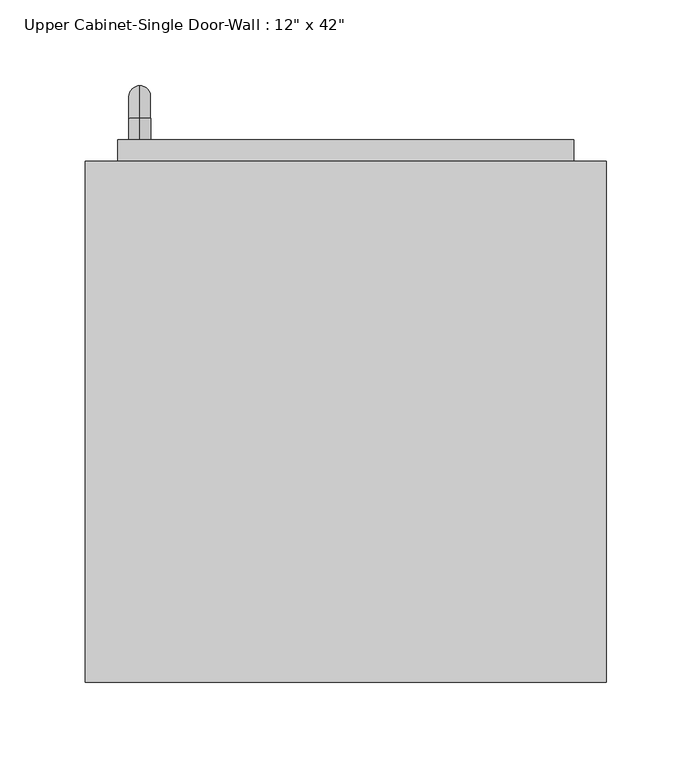
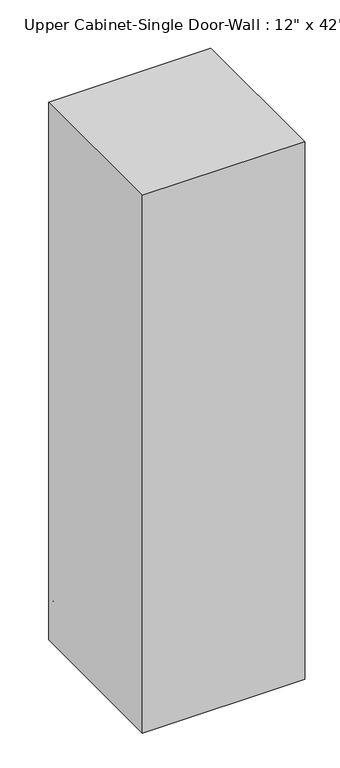
"""IFC4 building model written with IfcOpenShell, lengths in millimetres: furniture geometry."""

from ifc_helpers import new_model, si_unit, point, frame, origin, place, context, project, spatial, polyline, circle_curve, ellipse_curve, trimmed, outline, extrude, faceted_brep, source, transform, mapped, element, save
from ifc_brep_helpers import plane_surface, cylinder_surface, revolved_surface, advanced_brep


def furniture_aa269a34(model_context):
    return source(origin(), model_context, "Body", "SolidModel", [
        faceted_brep([(-122.6288372, 80.9625, 2438.4), (-122.6288372, 80.9625, 1371.6), (182.1711628, 80.9625, 1371.6), (182.1711628, 80.9625, 2438.4), (-122.6288372, 385.7625, 2438.4), (182.1711628, 385.7625, 2438.4), (182.1711628, 385.7625, 1371.6), (-122.6288372, 385.7625, 1371.6), (-103.5788372, 385.7625, 2419.35), (-103.5788372, 385.7625, 1390.65), (163.1211628, 385.7625, 1390.65), (163.1211628, 385.7625, 2419.35), (163.1211628, 100.0125, 2419.35), (-103.5788372, 100.0125, 2419.35), (163.1211628, 100.0125, 1390.65), (-103.5788372, 100.0125, 1390.65)], [[[0, 1, 2, 3]], [[4, 5, 6, 7], [8, 9, 10, 11]], [[1, 0, 4, 7]], [[2, 1, 7, 6]], [[3, 2, 6, 5]], [[0, 3, 5, 4]], [[8, 11, 12, 13]], [[11, 10, 14, 12]], [[10, 9, 15, 14]], [[9, 8, 13, 15]], [[13, 12, 14, 15]]]),
        advanced_brep(
        [(-90.8788372, 398.4625, 1517.65), (-90.8788372, 398.4625, 1530.35), (-90.8788372, 411.1625, 1517.65), (-90.8788372, 411.1625, 1530.35), (-90.8788372, 430.2125, 1511.3), (-90.8788372, 417.5125, 1511.3), (-90.8788372, 417.5125, 1435.1), (-90.8788372, 430.2125, 1435.1), (-90.8788372, 411.1625, 1416.05), (-90.8788372, 411.1625, 1428.75), (-90.8788372, 398.4625, 1428.75), (-90.8788372, 398.4625, 1416.05)],
        [
            (0, 1, circle_curve(frame((-90.8788372, 398.4625, 1524.0), z_axis=(0.0, -1.0, 0.0), x_axis=(0.0, 0.0, 1.0)), 6.35)),
            (1, 0, circle_curve(frame((-90.8788372, 398.4625, 1524.0), z_axis=(0.0, -1.0, 0.0), x_axis=(0.0, 0.0, 1.0)), 6.35)),
            (0, 2),
            (2, 3, circle_curve(frame((-90.8788372, 411.1625, 1524.0), z_axis=(0.0, -1.0, 0.0), x_axis=(0.0, 0.0, 1.0)), 6.35)),
            (3, 1),
            (3, 2, circle_curve(frame((-90.8788372, 411.1625, 1524.0), z_axis=(0.0, -1.0, 0.0), x_axis=(0.0, 0.0, 1.0)), 6.35)),
            (4, 3, circle_curve(frame((-90.8788372, 411.1625, 1511.3), z_axis=(1.0, 0.0, 0.0), x_axis=(0.0, 0.0, 1.0)), 19.05)),
            (2, 5, circle_curve(frame((-90.8788372, 411.1625, 1511.3), z_axis=(-1.0, 0.0, 0.0), x_axis=(0.0, 0.0, 1.0)), 6.35)),
            (5, 4, circle_curve(frame((-90.8788372, 423.8625, 1511.3), z_axis=(0.0, 0.0, 1.0), x_axis=(0.0, 1.0, 0.0)), 6.35)),
            (4, 5, circle_curve(frame((-90.8788372, 423.8625, 1511.3), z_axis=(0.0, 0.0, 1.0), x_axis=(0.0, 1.0, 0.0)), 6.35)),
            (5, 6),
            (6, 7, circle_curve(frame((-90.8788372, 423.8625, 1435.1), z_axis=(0.0, 0.0, 1.0), x_axis=(0.0, 1.0, 0.0)), 6.35)),
            (7, 4),
            (7, 6, circle_curve(frame((-90.8788372, 423.8625, 1435.1), z_axis=(0.0, 0.0, 1.0), x_axis=(0.0, 1.0, 0.0)), 6.35)),
            (8, 7, circle_curve(frame((-90.8788372, 411.1625, 1435.1), z_axis=(1.0, 0.0, 0.0), x_axis=(0.0, 1.0, 0.0)), 19.05)),
            (6, 9, circle_curve(frame((-90.8788372, 411.1625, 1435.1), z_axis=(-1.0, 0.0, 0.0), x_axis=(0.0, 1.0, 0.0)), 6.35)),
            (9, 8, circle_curve(frame((-90.8788372, 411.1625, 1422.4), z_axis=(0.0, 1.0, 0.0), x_axis=(0.0, 0.0, -1.0)), 6.35)),
            (8, 9, circle_curve(frame((-90.8788372, 411.1625, 1422.4), z_axis=(0.0, 1.0, 0.0), x_axis=(0.0, 0.0, -1.0)), 6.35)),
            (10, 11, circle_curve(frame((-90.8788372, 398.4625, 1422.4), z_axis=(0.0, -1.0, 0.0), x_axis=(0.0, 0.0, -1.0)), 6.35)),
            (11, 10, circle_curve(frame((-90.8788372, 398.4625, 1422.4), z_axis=(0.0, -1.0, 0.0), x_axis=(0.0, 0.0, -1.0)), 6.35)),
            (9, 10),
            (11, 8),
        ],
        [
            plane_surface(frame((-97.2288372, 398.4625, 1524.0), z_axis=(0.0, -1.0, 0.0), x_axis=(0.0, 0.0, 1.0))),
            cylinder_surface(frame((-90.8788372, 398.4625, 1524.0), z_axis=(0.0, -1.0, 0.0), x_axis=(0.0, 0.0, 1.0)), 6.35),
            revolved_surface(trimmed(ellipse_curve(frame((-90.8788372, 411.1625, 1524.0), z_axis=(0.0, -1.0, 0.0), x_axis=(0.0, 0.0, 1.0)), 6.35, 6.35), [point((-90.8788372, 411.1625, 1517.65))], [point((-90.8788372, 411.1625, 1530.35))], True, "CARTESIAN"), (-90.8788372, 411.1625, 1511.3), (-1.0, 0.0, 0.0)),
            revolved_surface(trimmed(ellipse_curve(frame((-90.8788372, 411.1625, 1524.0), z_axis=(0.0, -1.0, 0.0), x_axis=(0.0, 0.0, 1.0)), 6.35, 6.35), [point((-90.8788372, 411.1625, 1530.35))], [point((-90.8788372, 411.1625, 1517.65))], True, "CARTESIAN"), (-90.8788372, 411.1625, 1511.3), (-1.0, 0.0, 0.0)),
            cylinder_surface(frame((-90.8788372, 423.8625, 1511.3), z_axis=(0.0, 0.0, 1.0), x_axis=(0.0, 1.0, 0.0)), 6.35),
            revolved_surface(trimmed(ellipse_curve(frame((-90.8788372, 423.8625, 1435.1), z_axis=(0.0, 0.0, 1.0), x_axis=(0.0, 1.0, 0.0)), 6.35, 6.35), [point((-90.8788372, 417.5125, 1435.1))], [point((-90.8788372, 430.2125, 1435.1))], True, "CARTESIAN"), (-90.8788372, 411.1625, 1435.1), (-1.0, 0.0, 0.0)),
            revolved_surface(trimmed(ellipse_curve(frame((-90.8788372, 423.8625, 1435.1), z_axis=(0.0, 0.0, 1.0), x_axis=(0.0, 1.0, 0.0)), 6.35, 6.35), [point((-90.8788372, 430.2125, 1435.1))], [point((-90.8788372, 417.5125, 1435.1))], True, "CARTESIAN"), (-90.8788372, 411.1625, 1435.1), (-1.0, 0.0, 0.0)),
            plane_surface(frame((-97.2288372, 398.4625, 1422.4), z_axis=(0.0, -1.0, 0.0), x_axis=(0.0, 0.0, -1.0))),
            cylinder_surface(frame((-90.8788372, 411.1625, 1422.4), z_axis=(0.0, 1.0, 0.0), x_axis=(0.0, 0.0, -1.0)), 6.35),
        ],
        [
            (0, [[1, 2]]),
            (1, [[-1, 3, 4, 5]]),
            (1, [[-2, -5, 6, -3]]),
            (2, [[7, -4, 8, 9]]),
            (3, [[-8, -6, -7, 10]]),
            (4, [[-9, 11, 12, 13]]),
            (4, [[-10, -13, 14, -11]]),
            (5, [[15, -12, 16, 17]]),
            (6, [[-16, -14, -15, 18]]),
            (7, [[19, 20]]),
            (8, [[-17, 21, -20, 22]]),
            (8, [[-18, -22, -19, -21]]),
        ],
    ),
        extrude(outline(polyline([(-103.5788372, 398.4625), (163.1211628, 398.4625), (163.1211628, 366.7125), (-103.5788372, 366.7125), (-103.5788372, 398.4625)])), frame((0.0, 0.0, 1390.65), z_axis=(0.0, 0.0, 1.0), x_axis=(1.0, 0.0, 0.0)), (0.0, 0.0, 1.0), 1028.7),
    ])


if __name__ == "__main__":
    model = new_model("IFC4")
    model_context = context("Model", 3, world=origin())
    ifc_project = project(units=[si_unit("LENGTHUNIT", "METRE", prefix="MILLI")], contexts=[model_context])
    site = spatial("IfcSite", under=ifc_project)
    building = spatial("IfcBuilding", under=site)
    placement = place(None, origin())
    furniture_shape = furniture_aa269a34(model_context)
    element("IfcFurniture", 1, ObjectType="Upper Cabinet-Single Door-Wall : 12\" x 42\"", at=placement, inside=building, context=model_context, shape_type="MappedRepresentation", body=[
        mapped(furniture_shape, transform((0.0, 0.0, 0.0), x_axis=(1.0, 0.0, 0.0), y_axis=(0.0, 1.0, 0.0), z_axis=(0.0, 0.0, 1.0))),
    ])
    save(model, "model.ifc")

# Revit data of these elements
# Type "Upper Cabinet-Single Door-Wall : 12\" x 42\""
#   COBie.Type.CreatedBy = "doug.wood@us.ibm.com"
#   COBie.Type.CreatedOn = "2016-04-14T02:07:23"
#   COBie.Type.Name = "Casework_Upper Cabinet-Single Door-Wall_12\" x 42\""
#   COBie.Type.Category = "23-40 35 17 47 11 : Kitchen Casework"
#   COBie.Type.Description = "Upper Cabinet-Single Door-Wall_12\" x 42\""
#   COBie.Type.Manufacturer = ""
#   COBie.Type.ModelNumber = ""
#   Assembly Code = "C1030410"
#   COBie.Type.ReplacementCost = 0
#   Depth = 1' - 0"
#   Height = 3' - 6"
#   Top Of Cabinet = 8' - 0"
#   Width = 1' - 0"
#   COBie.Type = no
#   Cabinet Material = none
#   Door/Drawer Material = none
#   Handle Material = Cabinets - Handles
# Element 1 (IfcFurniture, "Upper Cabinet-Single Door-Wall : 12\" x 42\"")
#   Materials on its faces: "Cabinets", "Cabinets - Handles"
# Materials
#   "Cabinets - Handles": class "Metal", colour RGB 57 57 57, transparency 0
#   "Cabinets": class "Miscellaneous", colour RGB 249 249 249, transparency 0
